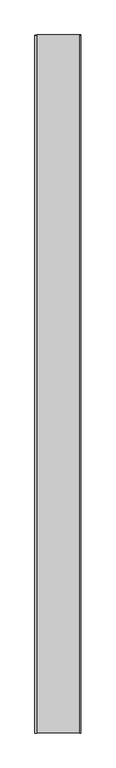
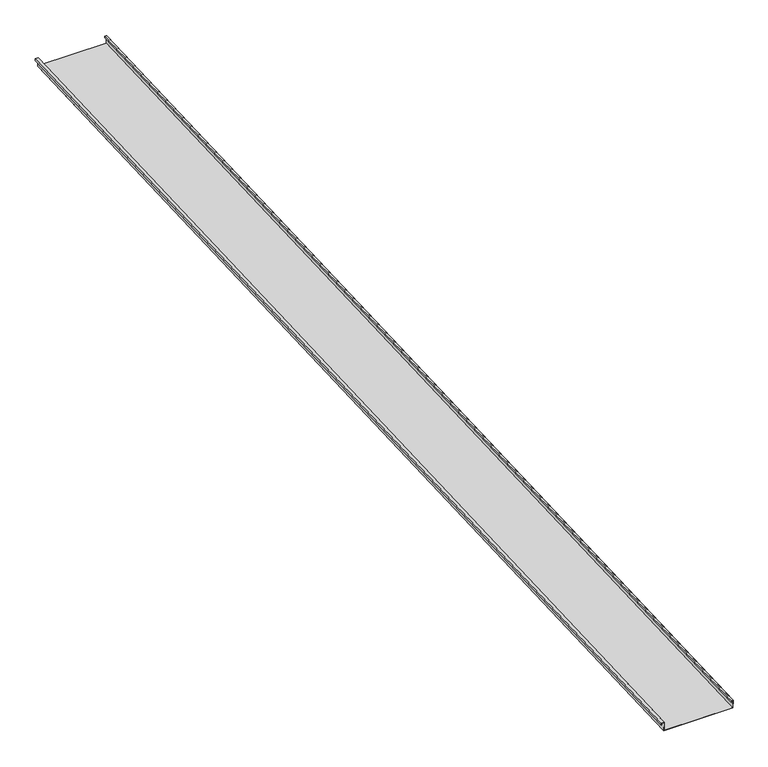
"""IFC4 building model written with IfcOpenShell, lengths in millimetres: proxy geometry, Generic Models 2:Generic Models 2:310765:Generic Models 2:310765 : Generic Models 2:Generic Models 2:310765:106 : Generic Models 2:Generic Models 2:310765:Generic Models 2:310765 : Generic Models 2:Generic Models 2:310765:300385."""

import ifcopenshell
import ifcopenshell.guid

model = None  # the IFC model being written
_history = None  # IfcOwnerHistory: only IFC2X3 demands one
_inside = {}  # id of a spatial element -> (the spatial element, [elements in it])
_under = {}  # id of a project, library or spatial element -> (it, [spatial elements below it])
_declared = {}  # id of a project -> (the project, [libraries it declares])
_typed = {}  # id of a type object -> (the type object, [elements of that type])
_made_of = {}  # id of a material, layer set ... -> (it, [elements and type objects made of it])


def new_model(schema):
    """Start an empty IFC model of exactly this schema.

    Asked for "IFC4X3", IfcOpenShell would pick the latest addendum, in which some entities
    have other attributes; the version numbers below select the first issue.
    IFC2X3 requires an IfcOwnerHistory on every rooted entity: one is made here for all.
    """
    global model, _history
    if schema == "IFC4X3":
        model = ifcopenshell.file(schema_version=(4, 3, 0, 0))
    else:
        model = ifcopenshell.file(schema=schema)
    _inside.clear()
    _under.clear()
    _declared.clear()
    _typed.clear()
    _made_of.clear()
    _history = None
    if model.schema == "IFC2X3":
        org = make("IfcOrganization", Name="unknown")
        user = make(
            "IfcPersonAndOrganization",
            ThePerson=make("IfcPerson", FamilyName="unknown"),
            TheOrganization=org,
        )
        app = make(
            "IfcApplication",
            ApplicationDeveloper=org,
            Version="unknown",
            ApplicationFullName="unknown",
            ApplicationIdentifier="unknown",
        )
        _history = make(
            "IfcOwnerHistory",
            OwningUser=user,
            OwningApplication=app,
            ChangeAction="ADDED",
            CreationDate=0,
        )
    return model


def make(cls, **values):
    """One entity of the class cls with the attributes given. An attribute that is None is left unset."""
    return model.create_entity(
        cls, **{name: value for name, value in values.items() if value is not None}
    )


def rooted(cls, **values):
    """An entity with a GlobalId (a new one), such as an element, a storey or a relation."""
    return make(cls, GlobalId=ifcopenshell.guid.new(), OwnerHistory=_history, **values)


def si_unit(unit_type, name, prefix=None):
    """IfcSIUnit, for example si_unit("LENGTHUNIT", "METRE", prefix="MILLI")."""
    return make("IfcSIUnit", UnitType=unit_type, Prefix=prefix, Name=name)


def assignment(units):
    """IfcUnitAssignment: the units of a project."""
    return None if units is None else make("IfcUnitAssignment", Units=units)


def point(xyz):
    """IfcCartesianPoint."""
    return None if xyz is None else make("IfcCartesianPoint", Coordinates=xyz)


def direction(xyz):
    """IfcDirection."""
    return None if xyz is None else make("IfcDirection", DirectionRatios=xyz)


def frame(location, z_axis=None, x_axis=None):
    """IfcAxis2Placement3D, a coordinate frame: its origin and axes. An axis left out is left unset."""
    return make(
        "IfcAxis2Placement3D",
        Location=point(location),
        Axis=direction(z_axis),
        RefDirection=direction(x_axis),
    )


def origin():
    """The frame at (0, 0, 0) with its axes left unset."""
    return frame((0.0, 0.0, 0.0))


def place(relative_to, where):
    """IfcLocalPlacement: puts the frame where relative to a parent placement (None: the world)."""
    return make(
        "IfcLocalPlacement", PlacementRelTo=relative_to, RelativePlacement=where
    )


def context(
    kind, dimensions, precision=None, world=None, true_north=None, identifier=None
):
    """IfcGeometricRepresentationContext, for example the 3D "Model" context."""
    return make(
        "IfcGeometricRepresentationContext",
        ContextIdentifier=identifier,
        ContextType=kind,
        CoordinateSpaceDimension=dimensions,
        Precision=precision,
        WorldCoordinateSystem=world,
        TrueNorth=true_north,
    )


def project(units=None, contexts=None):
    """IfcProject with its units and contexts."""
    return rooted(
        "IfcProject",
        Name="project",
        RepresentationContexts=contexts,
        UnitsInContext=assignment(units),
    )


def spatial(cls, under=None, at=None, **own):
    """A site, building, storey or space (cls), placed at a placement, below another one or the project."""
    s = rooted(cls, ObjectPlacement=at, **own)
    if under is not None:
        _under.setdefault(under.id(), (under, []))[1].append(s)
    return s


def polyline(points):
    """IfcPolyline through the points."""
    return make("IfcPolyline", Points=[point(p) for p in points])


def outline(outer, holes=None, kind="AREA"):
    """IfcArbitraryClosedProfileDef: a profile drawn as a closed curve; with holes, ...WithVoids."""
    if holes is None:
        return make("IfcArbitraryClosedProfileDef", ProfileType=kind, OuterCurve=outer)
    return make(
        "IfcArbitraryProfileDefWithVoids",
        ProfileType=kind,
        OuterCurve=outer,
        InnerCurves=holes,
    )


def extrude(swept, where, along, depth):
    """IfcExtrudedAreaSolid: the profile swept, set in the frame where, extruded along a direction by depth."""
    return make(
        "IfcExtrudedAreaSolid",
        SweptArea=swept,
        Position=where,
        ExtrudedDirection=direction(along),
        Depth=depth,
    )


def shape(context_of_items, identifier, shape_type, items):
    """IfcShapeRepresentation: the items that make up one representation, for example the "Body"."""
    return make(
        "IfcShapeRepresentation",
        ContextOfItems=context_of_items,
        RepresentationIdentifier=identifier,
        RepresentationType=shape_type,
        Items=items,
    )


def source(mapping_origin, context_of_items, identifier, shape_type, items):
    """IfcRepresentationMap: a shape defined once, which mapped items show again and again."""
    return make(
        "IfcRepresentationMap",
        MappingOrigin=mapping_origin,
        MappedRepresentation=shape(context_of_items, identifier, shape_type, items),
    )


def transform(
    local_origin,
    x_axis=None,
    y_axis=None,
    z_axis=None,
    scale=None,
    scale2=None,
    scale3=None,
    uniform=True,
):
    """IfcCartesianTransformationOperator3D, or its non-uniform kind. x_axis, y_axis, z_axis: its Axis1, 2, 3."""
    if uniform:
        return make(
            "IfcCartesianTransformationOperator3D",
            Axis1=direction(x_axis),
            Axis2=direction(y_axis),
            LocalOrigin=point(local_origin),
            Scale=scale,
            Axis3=direction(z_axis),
        )
    return make(
        "IfcCartesianTransformationOperator3DnonUniform",
        Axis1=direction(x_axis),
        Axis2=direction(y_axis),
        LocalOrigin=point(local_origin),
        Scale=scale,
        Axis3=direction(z_axis),
        Scale2=scale2,
        Scale3=scale3,
    )


def mapped(mapping_source, mapping_target):
    """IfcMappedItem: shows the shape of a source again, moved by a transform."""
    return make(
        "IfcMappedItem", MappingSource=mapping_source, MappingTarget=mapping_target
    )


def made_of(thing, what):
    """Note that an element or type object is made of a material, layer set ...; save() writes the relation."""
    if what is not None:
        _made_of.setdefault(what.id(), (what, []))[1].append(thing)
    return thing


def element(
    cls,
    number,
    at=None,
    inside=None,
    cuts=None,
    type_object=None,
    material=None,
    context=None,
    identifier="Body",
    shape_type=None,
    held_by="IfcProductDefinitionShape",
    body=None,
    shapes=None,
    **own,
):
    """One element of the class cls, such as IfcWall. Its Tag is "e" and its number.

    at: its placement. inside: the storey or other place that contains it. cuts: it is an
    opening in that element (IfcRelVoidsElement). A single representation is given by context,
    identifier, shape_type and body (its items); several are given by shapes. held_by: the class
    of the entity that holds the representations. save() writes the other relations.
    """
    e = rooted(cls, Tag="e%d" % number, ObjectPlacement=at, **own)
    if body is not None:
        shapes = [shape(context, identifier, shape_type, body)]
    if shapes is not None:
        e.Representation = make(held_by, Representations=shapes)
    if inside is not None:
        _inside.setdefault(inside.id(), (inside, []))[1].append(e)
    if cuts is not None:
        rooted(
            "IfcRelVoidsElement", RelatingBuildingElement=cuts, RelatedOpeningElement=e
        )
    if type_object is not None:
        _typed.setdefault(type_object.id(), (type_object, []))[1].append(e)
    return made_of(e, material)


def aggregate(whole, parts):
    """IfcRelAggregates: a whole, such as a stair, and the parts it consists of."""
    return rooted("IfcRelAggregates", RelatingObject=whole, RelatedObjects=parts)


def save(model, path):
    """Write the relations noted so far, then the file.

    IfcRelAggregates (storeys below a building ...), IfcRelContainedInSpatialStructure (elements
    in a storey), IfcRelDefinesByType, IfcRelAssociatesMaterial and IfcRelDeclares: one each for
    every whole, place, type object, material and project.
    """
    for whole, parts in _under.values():
        aggregate(whole, parts)
    for where, things in _inside.values():
        rooted(
            "IfcRelContainedInSpatialStructure",
            RelatedElements=things,
            RelatingStructure=where,
        )
    for kind, things in _typed.values():
        rooted("IfcRelDefinesByType", RelatedObjects=things, RelatingType=kind)
    for what, things in _made_of.values():
        rooted("IfcRelAssociatesMaterial", RelatedObjects=things, RelatingMaterial=what)
    for by, libraries in _declared.values():
        rooted("IfcRelDeclares", RelatingContext=by, RelatedDefinitions=libraries)
    model.write(path)


def generic_models_d265122d(model_context):
    return source(origin(), model_context, "Body", "SweptSolid", [
        extrude(outline(polyline([(1.5875, 0.0), (1.5875, 50.8), (407.9875, 50.8), (407.9875, 1.5875), (396.875, 1.5875), (396.875, 11.1125), (398.4625, 11.1125), (398.4625, 3.175), (406.4, 3.175), (406.4, 49.2125), (3.175, 49.2125), (3.175, -1.5874999), (-14.2875, -1.5874999), (-14.2875, 9.525), (-12.7, 9.525), (-12.7, 0.0), (1.5875, 0.0)])), frame((609876.8763073, -581354.4345603, 3902.6697972), z_axis=(0.0, 0.9991330730923568, 0.041630544712067834), x_axis=(1.0, 0.0, 0.0)), (0.0, 0.0, 1.0), 6400.8),
    ])


if __name__ == "__main__":
    model = new_model("IFC4")
    model_context = context("Model", 3, world=origin())
    ifc_project = project(units=[si_unit("LENGTHUNIT", "METRE", prefix="MILLI")], contexts=[model_context])
    site = spatial("IfcSite", under=ifc_project)
    building = spatial("IfcBuilding", under=site)
    placement = place(None, origin())
    generic_models_shape = generic_models_d265122d(model_context)
    element("IfcBuildingElementProxy", 1, Name="Generic Models 2:Generic Models 2:310765:Generic Models 2:310765 : Generic Models 2:Generic Models 2:310765:106 : Generic Models 2:Generic Models 2:310765:Generic Models 2:310765 : Generic Models 2:Generic Models 2:310765:300385", ObjectType="Generic Models 2:Generic Models 2:310765:Generic Models 2:310765 : Generic Models 2:Generic Models 2:310765:106 : Generic Models 2:Generic Models 2:310765:Generic Models 2:310765 : Generic Models 2:Generic Models 2:310765:300385", at=placement, inside=building, context=model_context, shape_type="MappedRepresentation", body=[
        mapped(generic_models_shape, transform((0.0, 0.0, 0.0), x_axis=(1.0, 0.0, 0.0), y_axis=(0.0, 1.0, 0.0), z_axis=(0.0, 0.0, 1.0))),
    ])
    save(model, "model.ifc")

# Revit data of these elements
# Type "Generic Models 2:Generic Models 2:310765:Generic Models 2:310765 : Generic Models 2:Generic Models 2:310765:106 : Generic Models 2:Generic Models 2:310765:Generic Models 2:310765 : Generic Models 2:Generic Models 2:310765:300385"
#   NameOverride = "Generic Models 2:Generic Models 2:310765:Generic Models 2:310765 : Generic Models 2:Generic Models 2:310765:300385"
#   ObjectTypeOverride = "Generic Models 2:310765 : Generic Models 2:Generic Models 2:310765"
#   Reference = "Generic Models 2"
#   Tag = "300385"
# Element 1 (IfcBuildingElementProxy, "Generic Models 2:Generic Models 2:310765:Generic Models 2:310765 : Generic Models 2:Generic Models 2:310765:106 : Generic Models 2:Generic Models 2:310765:Generic Models 2:310765 : Generic Models 2:Generic Models 2:310765:300385")
#   Materials on its faces: "THERMAL BROKEN ALUMINUM STOREFRONT FOR POLYCARBONATE"
# Materials
#   "THERMAL BROKEN ALUMINUM STOREFRONT FOR POLYCARBONATE": class "Unassigned", colour RGB 244 244 244, transparency 0, Keynote = "M07611300.01", Cost = 0
